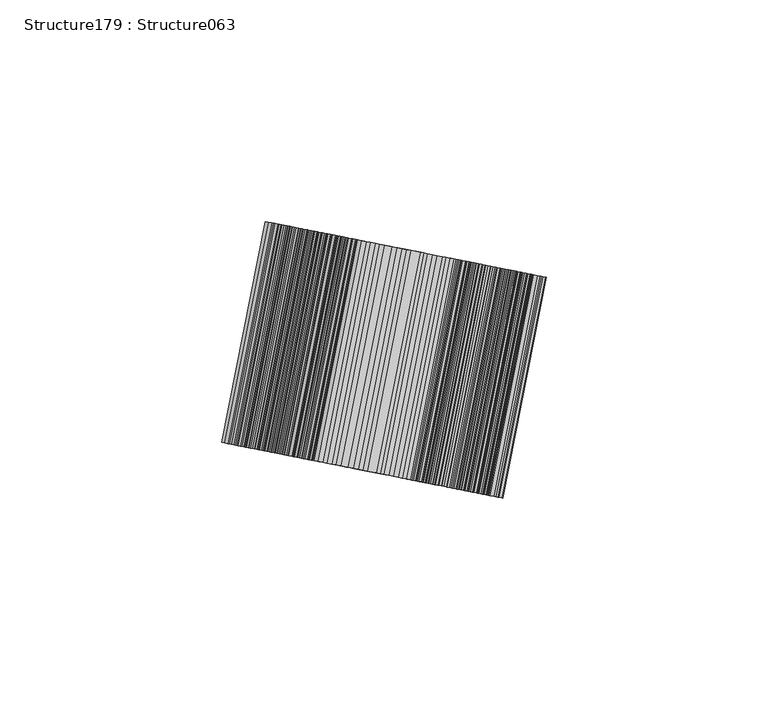
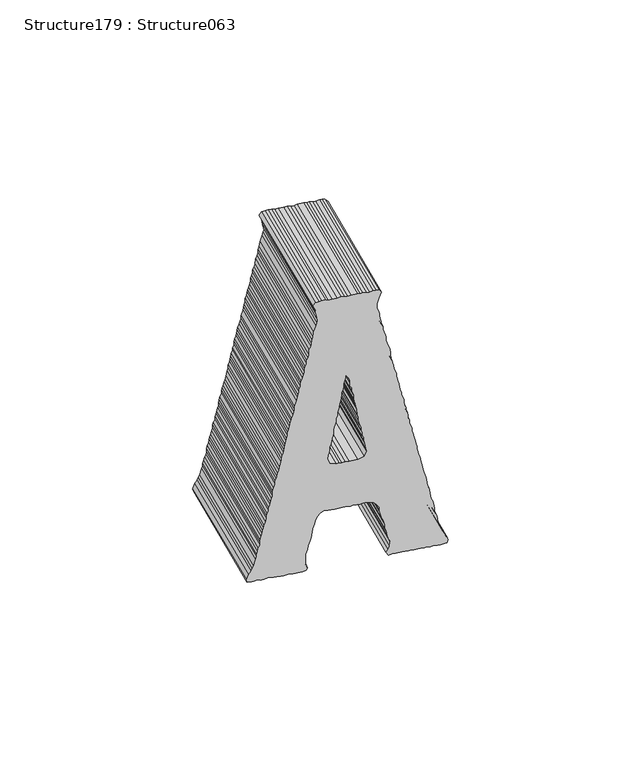
"""IFC4 building model written with IfcOpenShell, lengths in millimetres: proxy geometry, Structure179 : Structure063."""

from ifc_helpers import new_model, si_unit, frame, origin, place, context, project, spatial, polyline, outline, extrude, source, transform, mapped, element, save


def structure179_structure063_d8f3184d(model_context):
    return source(origin(), model_context, "Body", "SweptSolid", [
        extrude(outline(polyline([(0.9094651, 0.0), (2.0811665, -0.5187795), (2.9906316, -0.6522104), (4.1562841, -0.7806599), (5.1991801, -1.1663642), (5.9748585, -1.299795), (7.1504738, -1.6901249), (8.1894559, -1.6901249), (9.3551084, -2.0804549), (10.2645735, -2.3373539), (11.4362748, -2.5992343), (12.3453841, -2.8564891), (13.3818755, -2.9849386), (14.1582655, -3.3752685), (15.4626861, -3.5086994), (16.3721513, -3.5086994), (17.5385154, -3.7705798), (19.491944, -4.4131831), (20.2718921, -4.6750635), (21.3101626, -4.9369439), (22.3470097, -4.9369439), (23.2561191, -5.1988244), (24.4278204, -5.5891542), (25.4700048, -5.9745027), (26.6363689, -5.9745027), (27.4124031, -6.3651884), (28.7175354, -6.6270689), (30.535754, -7.0173988), (31.5743802, -7.1458483), (32.7400327, -7.4077287), (33.6555467, -7.7934329), (35.4741211, -7.7934329), (36.5102567, -7.5361781), (37.5492387, -7.2742978), (38.3288311, -6.8839679), (39.3671015, -6.3651884), (40.4099976, -7.2742978), (40.5395145, -8.1837628), (40.5395145, -9.0978536), (40.2826155, -10.2642177), (40.2826155, -11.3021323), (40.5395145, -12.473122), (40.4099976, -13.2491563), (40.5395145, -14.1632469), (40.5395145, -16.2390762), (40.2826155, -17.2816164), (40.2826155, -18.3195311), (40.5395145, -19.4858951), (40.4099976, -20.6618663), (40.4099976, -22.3470098), (40.2826155, -23.5183553), (40.5395145, -24.4228391), (40.5395145, -25.5988102), (40.4099976, -26.5032939), (40.2826155, -27.669658), (39.2382962, -28.4552992), (38.3288311, -27.9315384), (37.4197218, -27.669658), (36.6397736, -27.5458341), (35.4741211, -27.2839536), (33.5199809, -26.8936237), (32.6112274, -27.1555041), (31.4448633, -27.4173846), (29.3636968, -28.1934188), (27.545834, -28.4552992), (26.5089869, -28.7121982), (25.3372855, -28.8456292), (24.2943895, -29.1025281), (23.2561191, -29.6216633), (21.3101626, -29.7501128), (20.2718921, -30.0119932), (19.491944, -30.5357541), (18.3202426, -30.5357541), (17.2816164, -30.9214584), (16.3721513, -31.1783574), (15.3356599, -31.1783574), (14.1582655, -31.4402377), (13.1253323, -31.8305676), (12.2158672, -32.2208976), (11.4362748, -32.3543285), (10.2645735, -32.482778), (9.3551083, -32.8684823), (8.1894559, -32.8684823), (7.1504738, -33.2588122), (6.2374505, -33.392243), (5.0714422, -33.649142), (3.2475306, -34.2967268), (2.0811665, -34.2967268), (1.1720572, -34.5586072), (0.1334309, -34.8204876), (-1.0382704, -35.3392671), (-1.8178628, -35.472698), (-2.8568449, -35.7295969), (-3.8990293, -35.8630278), (-5.0653934, -36.2487321), (-5.8471206, -36.5106125), (-7.0166871, -36.5106125), (-8.1826954, -36.9009425), (-8.9644226, -37.029392), (-10.1364798, -37.4197219), (-11.1690572, -37.5485272), (-12.2115974, -37.6769767), (-12.9915456, -37.938857), (-14.03373, -38.329187), (-15.3292552, -38.4576365), (-16.3678815, -38.7195169), (-18.1861001, -39.1098468), (-19.3581573, -39.3671016), (-20.2672666, -39.7574314), (-21.4371888, -40.0143304), (-22.2189161, -40.2762109), (-23.1223323, -40.5380913), (-24.1648726, -40.5380913), (-25.465735, -41.0522451), (-26.5025822, -41.3141255), (-27.4173846, -41.4475564), (-28.4560108, -41.4475564), (-29.235959, -41.7044554), (-30.5311284, -42.0947853), (-31.3110766, -42.2282162), (-32.3536168, -42.6139205), (-33.5214042, -42.6139205), (-34.4308693, -43.1326999), (-35.3399786, -43.3945804), (-36.37647, -43.3945804), (-37.5424783, -43.6564608), (-38.7202285, -44.0467906), (-39.6236447, -44.3040454), (-40.405372, -44.5609444), (-41.5752942, -44.6943753), (-42.6139205, -45.0847053), (-43.7856218, -45.3465857), (-44.8221132, -45.3465857), (-45.7372714, -45.4750352), (-46.6406876, -45.989189), (-47.812389, -46.2510694), (-48.8510152, -46.5129498), (-49.7601245, -46.5129498), (-50.6731478, -46.9032797), (-52.8777823, -47.5508644), (-53.7929405, -47.9411943), (-54.5689747, -48.3315243), (-55.738897, -49.1125398), (-57.5532016, -49.7597688), (-58.4665807, -49.4978883), (-58.5957419, -48.2030748), (-58.4665807, -47.4270405), (-58.3331498, -46.2510694), (-58.5957419, -45.2131548), (-58.5957419, -44.0467906), (-58.3331498, -43.0042504), (-58.3331498, -42.0947853), (-58.4665807, -41.0522451), (-58.4665807, -40.1477614), (-58.5957419, -38.8479664), (-58.5957419, -37.938857), (-58.4665807, -36.9009425), (-58.3331498, -35.7295969), (-58.5957419, -34.8204876), (-58.5957419, -31.8305676), (-58.3331498, -30.6642036), (-57.4297336, -30.1404427), (-56.6480063, -30.5357541), (-55.6115149, -30.7926531), (-53.3972734, -30.7926531), (-52.3586471, -30.7926531), (-51.4495378, -30.5357541), (-50.6731478, -30.1404427), (-49.3683714, -30.0119932), (-48.4592621, -29.7501128), (-47.5497969, -29.3597829), (-46.6406876, -29.1025281), (-45.6038405, -28.8456292), (-43.2661308, -28.5837487), (-41.5752943, -27.9315384), (-40.2762109, -27.669658), (-38.9767716, -27.0270546), (-38.1950444, -26.112964), (-37.4190102, -24.6847195), (-37.6759092, -23.6468048), (-37.6759092, -21.56635), (-37.5424783, -20.266555), (-37.5424783, -17.5434969), (-37.6759092, -16.3675257), (-37.4190102, -15.463042), (-37.5424783, -14.4205017), (-37.6759092, -13.3825872), (-37.5424783, -12.473122), (-37.4190102, -11.1736828), (-37.6759092, -10.3926672), (-38.0676623, -8.8359732), (-38.8476105, -8.0553133), (-40.2762109, -7.0173988), (-41.4422191, -7.0173988), (-42.6139205, -6.7555184), (-44.5616561, -6.2367389), (-45.3472973, -5.7176037), (-46.5133056, -5.4557234), (-47.2932538, -5.3272739), (-48.33188, -5.3272739), (-49.3683714, -4.803513), (-50.4126907, -4.6750635), (-51.4495378, -4.546614), (-52.3586471, -4.1609097), (-53.6595096, -3.7705798), (-55.3489229, -3.8990293), (-56.6480063, -4.2893592), (-57.2966585, -4.9369439), (-58.5957419, -4.1609097), (-58.4665807, -2.9849386), (-58.3331498, -1.9470239), (-58.3331498, 0.1334309), (-58.4665807, 1.166364), (-58.4665807, 2.2092601), (-58.3331498, 3.1183694), (-58.4665807, 4.0328159), (-58.4665807, 5.3272737), (-58.3331498, 6.1082894), (-58.4665807, 7.403103), (-58.3331498, 8.1837628), (-58.5957419, 9.2216774), (-58.3331498, 10.3976485), (-58.5957419, 11.5640127), (-58.4665807, 12.4734778), (-58.3331498, 13.516018), (-58.3331498, 14.5489512), (-57.2966585, 14.9442625), (-56.3875492, 14.6823821), (-55.738897, 14.0301717), (-54.5689747, 13.7732728), (-53.7929405, 13.3825871), (-52.6151903, 12.8638077), (-50.6731478, 11.9543425), (-49.8875066, 11.6924621), (-48.5941162, 11.5640127), (-47.5497969, 11.3021323), (-46.6406876, 11.0452333), (-45.8646534, 10.6549033), (-44.5616561, 10.5264538), (-42.6139205, 10.2642176), (-41.4422191, 9.8738877), (-40.5384471, 9.4835579), (-39.6236447, 9.2216774), (-38.4576364, 9.0932279), (-37.4190102, 8.9697599), (-36.5059869, 8.8363289), (-35.6004358, 8.3171937), (-34.2956593, 8.1837628), (-33.3922431, 8.0553133), (-32.3536168, 7.9268638), (-31.4405935, 7.5365338), (-30.4019673, 7.146204), (-29.235959, 6.8889492), (-27.5447666, 6.6270688), (-26.3752002, 6.2367389), (-25.203143, 6.1082894), (-24.4235506, 5.8464089), (-23.3849244, 5.4607046), (-22.4793732, 5.3272737), (-21.3037579, 4.9369439), (-20.2672666, 4.9369439), (-19.3581573, 4.6750634), (-18.319531, 4.4181644), (-17.1474738, 4.156284), (-15.2018732, 3.6371488), (-14.1632469, 3.3802498), (-13.1207067, 3.3802498), (-12.2115974, 2.9899199), (-11.3024881, 2.59959), (-10.0012698, 2.59959), (-9.2270147, 2.0804548), (-8.1826954, 2.0804548), (-7.0166871, 1.9520053), (-5.9745027, 1.4282444), (-5.0653934, 1.4282444), (-4.1619771, 0.9094651), (-2.8568449, 0.7760342), (-1.9473797, 0.7760342), (-0.7817273, 0.2618804), (0.0, 0.0), (0.9094651, 0.0)]), holes=[polyline([(-20.9137838, -13.9013665), (-20.9137838, -16.8912865), (-20.7903157, -18.0576507), (-21.0472147, -19.2286403), (-20.7903157, -20.1381055), (-20.9137838, -21.0475706), (-20.2672666, -22.9945945), (-18.5817672, -23.6468048), (-17.2809048, -23.3849244), (-16.3678815, -23.1280254), (-15.4623303, -22.866145), (-14.1632469, -22.9945945), (-13.2480888, -22.4804408), (-12.2115974, -22.3470098), (-11.3024881, -22.2185603), (-10.393023, -21.8282304), (-9.3508386, -21.6947995), (-8.3122123, -21.6947995), (-7.146204, -21.56635), (-6.3644768, -21.1760201), (-5.3276296, -20.9187653), (-4.2854452, -20.9187653), (-3.117302, -20.3999858), (-1.9473797, -20.3999858), (-1.0382704, -20.009656), (-0.2561874, -19.8762251), (1.0389821, -19.7477756), (2.0811665, -19.4858951), (3.1180136, -19.2286403), (4.0274787, -19.1001908), (5.0714422, -19.1001908), (6.1082894, -18.5814114), (7.0177545, -18.4479805), (8.1894559, -18.4479805), (9.2216774, -18.0576507), (10.1368356, -17.7957702), (11.0463007, -17.7957702), (10.1368356, -17.1531669), (9.0928721, -16.7578556), (8.056025, -16.6294061), (6.8900167, -16.6294061), (6.1082894, -16.1106267), (4.9365881, -15.9771958), (3.1180136, -15.463042), (1.8189302, -15.3296111), (0.9094651, -15.2011616), (0.0, -14.9392812), (-1.0382704, -14.8108317), (-2.2078369, -14.4205017), (-4.2854452, -14.2870708), (-5.3276296, -14.0347974), (-6.3644768, -13.9013665), (-8.1826954, -13.5110367), (-9.2270147, -12.9922573), (-10.2638619, -12.9922573), (-11.1690572, -12.7303768), (-12.3446725, -12.6015715), (-13.1207067, -12.216223), (-14.286715, -12.216223), (-15.4623303, -11.8209118), (-17.2809048, -11.5640128), (-18.5817672, -11.3021323), (-20.1377496, -12.0827921), (-20.9137838, -13.9013665)])]), frame((-2601.9221634, 234984.851897, 444.9951864), z_axis=(0.19466222296394123, 0.9808703374813295, 0.0), x_axis=(0.0, 0.0, 1.0)), (0.0, 0.0, 1.0), 50.8),
    ])


if __name__ == "__main__":
    model = new_model("IFC4")
    model_context = context("Model", 3, world=origin())
    ifc_project = project(units=[si_unit("LENGTHUNIT", "METRE", prefix="MILLI")], contexts=[model_context])
    site = spatial("IfcSite", under=ifc_project)
    building = spatial("IfcBuilding", under=site)
    placement = place(None, origin())
    structure179_structure063_shape = structure179_structure063_d8f3184d(model_context)
    element("IfcBuildingElementProxy", 1, Name="Structure179 : Structure063", ObjectType="Structure179 : Structure063", at=placement, inside=building, context=model_context, shape_type="MappedRepresentation", body=[
        mapped(structure179_structure063_shape, transform((0.0, 0.0, 0.0), x_axis=(1.0, 0.0, 0.0), y_axis=(0.0, 1.0, 0.0), z_axis=(0.0, 0.0, 1.0))),
    ])
    save(model, "model.ifc")

# Revit data of these elements
# Type "Structure179 : Structure063"
#   NameOverride = "Structure063"
# Element 1 (IfcBuildingElementProxy, "Structure179 : Structure063")
#   Materials on its faces: "BRUSHED ALUMINUM LETTERING"
# Materials
#   "BRUSHED ALUMINUM LETTERING": class "Unassigned", colour RGB 169 181 186, transparency 0, Cost = 0
